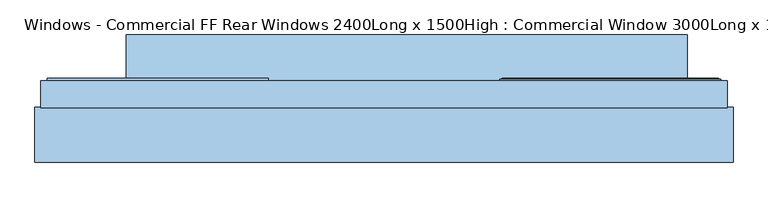
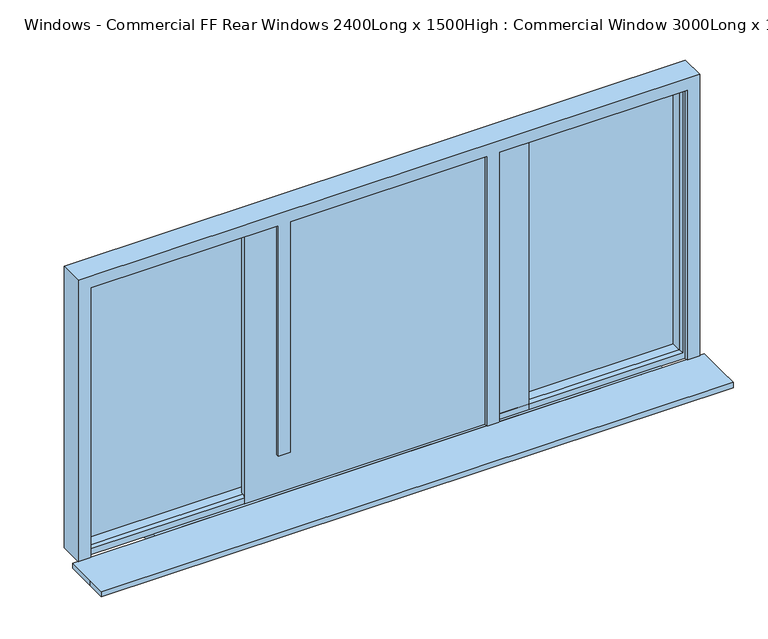
"""IFC4 building model written with IfcOpenShell, lengths in millimetres: window geometry, Windows - Commercial FF Rear Windows 2400Long x 1500High : Commercial Window 3000Long x 1500High 2."""

import ifcopenshell
import ifcopenshell.guid

model = None  # the IFC model being written
_history = None  # IfcOwnerHistory: only IFC2X3 demands one
_inside = {}  # id of a spatial element -> (the spatial element, [elements in it])
_under = {}  # id of a project, library or spatial element -> (it, [spatial elements below it])
_declared = {}  # id of a project -> (the project, [libraries it declares])
_typed = {}  # id of a type object -> (the type object, [elements of that type])
_made_of = {}  # id of a material, layer set ... -> (it, [elements and type objects made of it])


def new_model(schema):
    """Start an empty IFC model of exactly this schema.

    Asked for "IFC4X3", IfcOpenShell would pick the latest addendum, in which some entities
    have other attributes; the version numbers below select the first issue.
    IFC2X3 requires an IfcOwnerHistory on every rooted entity: one is made here for all.
    """
    global model, _history
    if schema == "IFC4X3":
        model = ifcopenshell.file(schema_version=(4, 3, 0, 0))
    else:
        model = ifcopenshell.file(schema=schema)
    _inside.clear()
    _under.clear()
    _declared.clear()
    _typed.clear()
    _made_of.clear()
    _history = None
    if model.schema == "IFC2X3":
        org = make("IfcOrganization", Name="unknown")
        user = make(
            "IfcPersonAndOrganization",
            ThePerson=make("IfcPerson", FamilyName="unknown"),
            TheOrganization=org,
        )
        app = make(
            "IfcApplication",
            ApplicationDeveloper=org,
            Version="unknown",
            ApplicationFullName="unknown",
            ApplicationIdentifier="unknown",
        )
        _history = make(
            "IfcOwnerHistory",
            OwningUser=user,
            OwningApplication=app,
            ChangeAction="ADDED",
            CreationDate=0,
        )
    return model


def make(cls, **values):
    """One entity of the class cls with the attributes given. An attribute that is None is left unset."""
    return model.create_entity(
        cls, **{name: value for name, value in values.items() if value is not None}
    )


def rooted(cls, **values):
    """An entity with a GlobalId (a new one), such as an element, a storey or a relation."""
    return make(cls, GlobalId=ifcopenshell.guid.new(), OwnerHistory=_history, **values)


def si_unit(unit_type, name, prefix=None):
    """IfcSIUnit, for example si_unit("LENGTHUNIT", "METRE", prefix="MILLI")."""
    return make("IfcSIUnit", UnitType=unit_type, Prefix=prefix, Name=name)


def assignment(units):
    """IfcUnitAssignment: the units of a project."""
    return None if units is None else make("IfcUnitAssignment", Units=units)


def point(xyz):
    """IfcCartesianPoint."""
    return None if xyz is None else make("IfcCartesianPoint", Coordinates=xyz)


def direction(xyz):
    """IfcDirection."""
    return None if xyz is None else make("IfcDirection", DirectionRatios=xyz)


def frame(location, z_axis=None, x_axis=None):
    """IfcAxis2Placement3D, a coordinate frame: its origin and axes. An axis left out is left unset."""
    return make(
        "IfcAxis2Placement3D",
        Location=point(location),
        Axis=direction(z_axis),
        RefDirection=direction(x_axis),
    )


def origin():
    """The frame at (0, 0, 0) with its axes left unset."""
    return frame((0.0, 0.0, 0.0))


def place(relative_to, where):
    """IfcLocalPlacement: puts the frame where relative to a parent placement (None: the world)."""
    return make(
        "IfcLocalPlacement", PlacementRelTo=relative_to, RelativePlacement=where
    )


def context(
    kind, dimensions, precision=None, world=None, true_north=None, identifier=None
):
    """IfcGeometricRepresentationContext, for example the 3D "Model" context."""
    return make(
        "IfcGeometricRepresentationContext",
        ContextIdentifier=identifier,
        ContextType=kind,
        CoordinateSpaceDimension=dimensions,
        Precision=precision,
        WorldCoordinateSystem=world,
        TrueNorth=true_north,
    )


def project(units=None, contexts=None):
    """IfcProject with its units and contexts."""
    return rooted(
        "IfcProject",
        Name="project",
        RepresentationContexts=contexts,
        UnitsInContext=assignment(units),
    )


def spatial(cls, under=None, at=None, **own):
    """A site, building, storey or space (cls), placed at a placement, below another one or the project."""
    s = rooted(cls, ObjectPlacement=at, **own)
    if under is not None:
        _under.setdefault(under.id(), (under, []))[1].append(s)
    return s


def polyline(points):
    """IfcPolyline through the points."""
    return make("IfcPolyline", Points=[point(p) for p in points])


def outline(outer, holes=None, kind="AREA"):
    """IfcArbitraryClosedProfileDef: a profile drawn as a closed curve; with holes, ...WithVoids."""
    if holes is None:
        return make("IfcArbitraryClosedProfileDef", ProfileType=kind, OuterCurve=outer)
    return make(
        "IfcArbitraryProfileDefWithVoids",
        ProfileType=kind,
        OuterCurve=outer,
        InnerCurves=holes,
    )


def extrude(swept, where, along, depth):
    """IfcExtrudedAreaSolid: the profile swept, set in the frame where, extruded along a direction by depth."""
    return make(
        "IfcExtrudedAreaSolid",
        SweptArea=swept,
        Position=where,
        ExtrudedDirection=direction(along),
        Depth=depth,
    )


def faces_of(points, faces, orient=None, outer=None):
    """IfcFace entities. A face is a list of loops; a loop is a list of indices into points, from 0.

    orient and outer hold one flag for each loop. By default every Orientation is true, the
    first loop of a face is its IfcFaceOuterBound and the others are IfcFaceBound.
    """
    made = []
    for i, loops in enumerate(faces):
        bounds = []
        for j, loop in enumerate(loops):
            is_outer = j == 0 if outer is None else outer[i][j]
            bounds.append(
                make(
                    "IfcFaceOuterBound" if is_outer else "IfcFaceBound",
                    Bound=make("IfcPolyLoop", Polygon=[points[k] for k in loop]),
                    Orientation=True if orient is None else orient[i][j],
                )
            )
        made.append(make("IfcFace", Bounds=bounds))
    return made


def faceted_brep(points, faces, orient=None, outer=None, voids=None):
    """IfcFacetedBrep: a solid bounded by flat faces; with voids (closed shells), ...WithVoids."""
    shared = [point(p) for p in points]
    hull = make("IfcClosedShell", CfsFaces=faces_of(shared, faces, orient, outer))
    if voids is None:
        return make("IfcFacetedBrep", Outer=hull)
    return make(
        "IfcFacetedBrepWithVoids",
        Outer=hull,
        Voids=[
            make(cls, CfsFaces=faces_of(shared, fs, o, b)) for cls, fs, o, b in voids
        ],
    )


def shape(context_of_items, identifier, shape_type, items):
    """IfcShapeRepresentation: the items that make up one representation, for example the "Body"."""
    return make(
        "IfcShapeRepresentation",
        ContextOfItems=context_of_items,
        RepresentationIdentifier=identifier,
        RepresentationType=shape_type,
        Items=items,
    )


def source(mapping_origin, context_of_items, identifier, shape_type, items):
    """IfcRepresentationMap: a shape defined once, which mapped items show again and again."""
    return make(
        "IfcRepresentationMap",
        MappingOrigin=mapping_origin,
        MappedRepresentation=shape(context_of_items, identifier, shape_type, items),
    )


def transform(
    local_origin,
    x_axis=None,
    y_axis=None,
    z_axis=None,
    scale=None,
    scale2=None,
    scale3=None,
    uniform=True,
):
    """IfcCartesianTransformationOperator3D, or its non-uniform kind. x_axis, y_axis, z_axis: its Axis1, 2, 3."""
    if uniform:
        return make(
            "IfcCartesianTransformationOperator3D",
            Axis1=direction(x_axis),
            Axis2=direction(y_axis),
            LocalOrigin=point(local_origin),
            Scale=scale,
            Axis3=direction(z_axis),
        )
    return make(
        "IfcCartesianTransformationOperator3DnonUniform",
        Axis1=direction(x_axis),
        Axis2=direction(y_axis),
        LocalOrigin=point(local_origin),
        Scale=scale,
        Axis3=direction(z_axis),
        Scale2=scale2,
        Scale3=scale3,
    )


def mapped(mapping_source, mapping_target):
    """IfcMappedItem: shows the shape of a source again, moved by a transform."""
    return make(
        "IfcMappedItem", MappingSource=mapping_source, MappingTarget=mapping_target
    )


def made_of(thing, what):
    """Note that an element or type object is made of a material, layer set ...; save() writes the relation."""
    if what is not None:
        _made_of.setdefault(what.id(), (what, []))[1].append(thing)
    return thing


def element(
    cls,
    number,
    at=None,
    inside=None,
    cuts=None,
    type_object=None,
    material=None,
    context=None,
    identifier="Body",
    shape_type=None,
    held_by="IfcProductDefinitionShape",
    body=None,
    shapes=None,
    **own,
):
    """One element of the class cls, such as IfcWall. Its Tag is "e" and its number.

    at: its placement. inside: the storey or other place that contains it. cuts: it is an
    opening in that element (IfcRelVoidsElement). A single representation is given by context,
    identifier, shape_type and body (its items); several are given by shapes. held_by: the class
    of the entity that holds the representations. save() writes the other relations.
    """
    e = rooted(cls, Tag="e%d" % number, ObjectPlacement=at, **own)
    if body is not None:
        shapes = [shape(context, identifier, shape_type, body)]
    if shapes is not None:
        e.Representation = make(held_by, Representations=shapes)
    if inside is not None:
        _inside.setdefault(inside.id(), (inside, []))[1].append(e)
    if cuts is not None:
        rooted(
            "IfcRelVoidsElement", RelatingBuildingElement=cuts, RelatedOpeningElement=e
        )
    if type_object is not None:
        _typed.setdefault(type_object.id(), (type_object, []))[1].append(e)
    return made_of(e, material)


def aggregate(whole, parts):
    """IfcRelAggregates: a whole, such as a stair, and the parts it consists of."""
    return rooted("IfcRelAggregates", RelatingObject=whole, RelatedObjects=parts)


def save(model, path):
    """Write the relations noted so far, then the file.

    IfcRelAggregates (storeys below a building ...), IfcRelContainedInSpatialStructure (elements
    in a storey), IfcRelDefinesByType, IfcRelAssociatesMaterial and IfcRelDeclares: one each for
    every whole, place, type object, material and project.
    """
    for whole, parts in _under.values():
        aggregate(whole, parts)
    for where, things in _inside.values():
        rooted(
            "IfcRelContainedInSpatialStructure",
            RelatedElements=things,
            RelatingStructure=where,
        )
    for kind, things in _typed.values():
        rooted("IfcRelDefinesByType", RelatedObjects=things, RelatingType=kind)
    for what, things in _made_of.values():
        rooted("IfcRelAssociatesMaterial", RelatedObjects=things, RelatingMaterial=what)
    for by, libraries in _declared.values():
        rooted("IfcRelDeclares", RelatingContext=by, RelatedDefinitions=libraries)
    model.write(path)


def windows_commercial_ff_rear_windows_2400long_x_1500high_ec56d910(model_context):
    return source(origin(), model_context, "Body", "SolidModel", [
        extrude(outline(polyline([(-2260.0, -231.5434322), (-2260.0, -138.5434322), (-2260.0, 8.4565678), (790.0, 8.4565678), (790.0, -138.5434322), (790.0, -231.5434322), (-2260.0, -231.5434322)])), frame((0.0, 0.0, 636.5715519), z_axis=(0.0, 0.0, 1.0), x_axis=(1.0, 0.0, 0.0)), (0.0, 0.0, 1.0), 26.4284481),
        extrude(outline(polyline([(695.0, 87.4565678), (-190.0, 87.4565678), (-190.0, 111.4565678), (695.0, 111.4565678), (695.0, 87.4565678)])), frame((0.0, 0.0, 693.0), z_axis=(0.0, 0.0, 1.0), x_axis=(1.0, 0.0, 0.0)), (0.0, 0.0, 1.0), 1337.0),
        extrude(outline(polyline([(-1420.0, 47.4565678), (-50.0, 47.4565678), (-50.0, 23.4565678), (-1420.0, 23.4565678), (-1420.0, 47.4565678)])), frame((0.0, 0.0, 663.0), z_axis=(0.0, 0.0, 1.0), x_axis=(1.0, 0.0, 0.0)), (0.0, 0.0, 1.0), 1397.0),
        extrude(outline(polyline([(-1280.0, 87.4565678), (-2165.0, 87.4565678), (-2165.0, 111.4565678), (-1280.0, 111.4565678), (-1280.0, 87.4565678)])), frame((0.0, 0.0, 693.0), z_axis=(0.0, 0.0, 1.0), x_axis=(1.0, 0.0, 0.0)), (0.0, 0.0, 1.0), 1337.0),
        faceted_brep([(-2235.0, 5.4565678, 663.0), (-2175.0, 5.4565678, 663.0), (-2175.0, 5.4565678, 2040.0), (-1268.0, 5.4565678, 2040.0), (-1268.0, 5.4565678, 863.0), (-1210.0, 5.4565678, 863.0), (-1210.0, 5.4565678, 2040.0), (-260.0, 5.4565678, 2040.0), (-260.0, 5.4565678, 663.0), (-202.0, 5.4565678, 663.0), (-202.0, 5.4565678, 2040.0), (705.0, 5.4565678, 2040.0), (705.0, 5.4565678, 663.0), (765.0, 5.4565678, 663.0), (765.0, 5.4565678, 2100.0), (-2235.0, 5.4565678, 2100.0), (-2235.0, 123.4565678, 663.0), (-2235.0, 123.4565678, 2100.0), (-2195.0, 123.4565678, 663.0), (765.0, 123.4565678, 2100.0), (765.0, 123.4565678, 663.0), (725.0, 123.4565678, 663.0), (725.0, 123.4565678, 2060.0), (-220.0, 123.4565678, 2060.0), (-220.0, 123.4565678, 663.0), (-260.0, 123.4565678, 663.0), (-260.0, 123.4565678, 2060.0), (-1210.0, 123.4565678, 2060.0), (-1210.0, 123.4565678, 863.0), (-1250.0, 123.4565678, 863.0), (-1250.0, 123.4565678, 2060.0), (-2195.0, 123.4565678, 2060.0), (-2195.0, 23.4565678, 663.0), (-2195.0, 23.4565678, 2060.0), (-2175.0, 23.4565678, 663.0), (-1250.0, 23.4565678, 2060.0), (-1250.0, 23.4565678, 863.0), (-1268.0, 23.4565678, 863.0), (-1268.0, 23.4565678, 2040.0), (-2175.0, 23.4565678, 2040.0), (725.0, 23.4565678, 2060.0), (725.0, 23.4565678, 663.0), (705.0, 23.4565678, 663.0), (705.0, 23.4565678, 2040.0), (-202.0, 23.4565678, 2040.0), (-202.0, 23.4565678, 663.0), (-220.0, 23.4565678, 663.0), (-220.0, 23.4565678, 2060.0), (-1210.0, 23.4565678, 863.0), (-1220.0, 23.4565678, 863.0), (-1220.0, 23.4565678, 2060.0), (-250.0, 23.4565678, 2060.0), (-250.0, 23.4565678, 663.0), (-260.0, 23.4565678, 663.0), (-260.0, 23.4565678, 2040.0), (-1210.0, 23.4565678, 2040.0), (-1210.0, 47.4565678, 2060.0), (-260.0, 47.4565678, 2060.0), (-250.0, 47.4565678, 2060.0), (-1220.0, 47.4565678, 2060.0), (-1210.0, 47.4565678, 863.0), (-1220.0, 47.4565678, 863.0), (-250.0, 47.4565678, 663.0), (-260.0, 47.4565678, 663.0), (-260.0, 73.4565678, 663.0), (-220.0, 73.4565678, 663.0), (-202.0, 8.4565678, 663.0), (-260.0, 8.4565678, 663.0), (590.0, 323.4565678, 600.0), (590.0, 8.4565678, 600.0), (-1860.0, 8.4565678, 600.0), (-1860.0, 323.4565678, 600.0), (590.0, 323.4565678, 637.0666405), (-1860.0, 323.4565678, 637.0666405), (590.0, 73.4565678, 649.0962075), (-1860.0, 73.4565678, 649.0962075), (590.0, 8.4565678, 663.0), (590.0, 73.4565678, 663.0), (-1860.0, 73.4565678, 663.0), (-1860.0, 8.4565678, 663.0)], [[[0, 1, 2, 3, 4, 5, 6, 7, 8, 9, 10, 11, 12, 13, 14, 15]], [[16, 0, 15, 17]], [[18, 16, 17, 19, 20, 21, 22, 23, 24, 25, 26, 27, 28, 29, 30, 31]], [[32, 18, 31, 33]], [[34, 32, 33, 35, 36, 37, 38, 39]], [[40, 41, 42, 43, 44, 45, 46, 47]], [[48, 49, 50, 51, 52, 53, 54, 55]], [[1, 34, 39, 2]], [[15, 14, 19, 17]], [[33, 31, 30, 35]], [[22, 40, 47, 23]], [[56, 27, 26, 57, 58, 51, 50, 59]], [[2, 39, 38, 3]], [[43, 11, 10, 44]], [[6, 55, 54, 7]], [[14, 13, 20, 19]], [[22, 21, 41, 40]], [[12, 11, 43, 42]], [[5, 48, 55, 6]], [[37, 4, 3, 38]], [[29, 36, 35, 30]], [[60, 28, 27, 56]], [[61, 60, 56, 59]], [[49, 61, 59, 50]], [[58, 62, 52, 51]], [[62, 58, 57, 63]], [[63, 57, 26, 25, 64]], [[24, 23, 47, 46, 65]], [[10, 9, 66, 45, 44]], [[8, 7, 54, 53, 67]], [[68, 69, 70, 71]], [[72, 68, 71, 73]], [[74, 72, 73, 75]], [[76, 77, 65, 46, 45, 66]], [[78, 79, 67, 53, 52, 62, 63, 64]], [[1, 0, 16, 18, 32, 34]], [[13, 12, 42, 41, 21, 20]], [[48, 5, 4, 37, 36, 29, 28, 60, 61, 49]], [[25, 24, 65, 64]], [[9, 8, 67, 66]], [[76, 69, 68, 72, 74, 77]], [[79, 78, 75, 73, 71, 70]], [[77, 74, 75, 78, 64, 65]], [[69, 76, 66, 67, 79, 70]]]),
        faceted_brep([(-1250.0, 23.4565678, 2060.0), (-1250.0, 93.4565678, 2060.0), (-2195.0, 93.4565678, 2060.0), (-2195.0, 23.4565678, 2060.0), (-1290.0, 37.9494677, 2020.0), (-1279.8519623, 23.4565678, 2030.1480377), (-2165.1480377, 23.4565678, 2030.1480377), (-2155.0, 37.9494677, 2020.0), (-1290.0, 87.4565678, 2020.0), (-2155.0, 87.4565678, 2020.0), (-1280.0, 111.4565678, 2030.0), (-1280.0, 87.4565678, 2030.0), (-2165.0, 87.4565678, 2030.0), (-2165.0, 111.4565678, 2030.0), (-1290.0, 129.2300705, 2020.0), (-1290.0, 111.4565678, 2020.0), (-2155.0, 111.4565678, 2020.0), (-2155.0, 129.2300705, 2020.0), (-1271.1854344, 135.0035732, 2038.8145656), (-2173.8145656, 135.0035732, 2038.8145656), (-2195.0, 93.4565678, 663.0), (-2195.0, 23.4565678, 663.0), (-2165.1480377, 23.4565678, 692.8519623), (-2155.0, 37.9494677, 703.0), (-2155.0, 87.4565678, 703.0), (-2165.0, 87.4565678, 693.0), (-2165.0, 111.4565678, 693.0), (-2155.0, 111.4565678, 703.0), (-2155.0, 129.2300705, 703.0), (-2173.8145656, 135.0035732, 684.1854344), (-1250.0, 93.4565678, 663.0), (-1250.0, 23.4565678, 663.0), (-1279.8519623, 23.4565678, 692.8519623), (-1290.0, 37.9494677, 703.0), (-1290.0, 87.4565678, 703.0), (-1280.0, 87.4565678, 693.0), (-1280.0, 111.4565678, 693.0), (-1290.0, 111.4565678, 703.0), (-1290.0, 129.2300705, 703.0), (-1271.1854344, 135.0035732, 684.1854344), (-1240.0, 135.0035732, 653.0), (-2205.0, 135.0035732, 653.0), (-2205.0, 135.0035732, 2070.0), (-1240.0, 135.0035732, 2070.0), (-1240.0, 93.4565678, 2070.0), (-2205.0, 93.4565678, 2070.0), (-2205.0, 93.4565678, 653.0), (-1240.0, 93.4565678, 653.0)], [[[0, 1, 2, 3]], [[4, 5, 6, 7]], [[8, 4, 7, 9]], [[10, 11, 12, 13]], [[14, 15, 16, 17]], [[18, 14, 17, 19]], [[3, 2, 20, 21]], [[7, 6, 22, 23]], [[9, 7, 23, 24]], [[13, 12, 25, 26]], [[17, 16, 27, 28]], [[19, 17, 28, 29]], [[21, 20, 30, 31]], [[0, 3, 21, 31], [32, 22, 6, 5]], [[23, 22, 32, 33]], [[24, 23, 33, 34]], [[35, 25, 12, 11], [8, 9, 24, 34]], [[26, 25, 35, 36]], [[10, 13, 26, 36], [37, 27, 16, 15]], [[28, 27, 37, 38]], [[29, 28, 38, 39]], [[40, 41, 42, 43], [18, 19, 29, 39]], [[30, 1, 0, 31]], [[33, 32, 5, 4]], [[34, 33, 4, 8]], [[36, 35, 11, 10]], [[38, 37, 15, 14]], [[39, 38, 14, 18]], [[44, 43, 42, 45]], [[45, 42, 41, 46]], [[46, 41, 40, 47]], [[47, 40, 43, 44]], [[45, 46, 47, 44], [1, 30, 20, 2]]]),
        faceted_brep([(-230.0, 87.4565678, 2070.0), (-230.0, 129.2300705, 2070.0), (-230.0, 129.2300705, 653.0), (-230.0, 87.4565678, 653.0), (-220.0, 23.4565678, 2060.0), (-220.0, 87.4565678, 2060.0), (-220.0, 87.4565678, 663.0), (-220.0, 23.4565678, 663.0), (-180.0, 37.9494677, 2020.0), (-190.1480377, 23.4565678, 2030.1480377), (-190.1480377, 23.4565678, 692.8519623), (-180.0, 37.9494677, 703.0), (-180.0, 87.4565678, 2020.0), (-180.0, 87.4565678, 703.0), (-190.0, 111.4565678, 2030.0), (-190.0, 87.4565678, 2030.0), (-190.0, 87.4565678, 693.0), (-190.0, 111.4565678, 693.0), (-180.0, 129.2300705, 2020.0), (-180.0, 111.4565678, 2020.0), (-180.0, 111.4565678, 703.0), (-180.0, 129.2300705, 703.0), (-197.4457548, 135.0035732, 2037.4457548), (-197.4457548, 135.0035732, 685.5542452), (-219.2153903, 135.0035732, 2059.2153903), (-219.2153903, 135.0035732, 663.7846097), (735.0, 129.2300705, 653.0), (735.0, 87.4565678, 653.0), (725.0, 87.4565678, 663.0), (725.0, 23.4565678, 663.0), (695.1480377, 23.4565678, 692.8519623), (685.0, 37.9494677, 703.0), (685.0, 87.4565678, 703.0), (695.0, 87.4565678, 693.0), (695.0, 111.4565678, 693.0), (685.0, 111.4565678, 703.0), (685.0, 129.2300705, 703.0), (702.4457548, 135.0035732, 685.5542452), (724.2153903, 135.0035732, 663.7846097), (735.0, 129.2300705, 2070.0), (735.0, 87.4565678, 2070.0), (725.0, 87.4565678, 2060.0), (725.0, 23.4565678, 2060.0), (695.1480377, 23.4565678, 2030.1480377), (685.0, 37.9494677, 2020.0), (685.0, 87.4565678, 2020.0), (695.0, 87.4565678, 2030.0), (695.0, 111.4565678, 2030.0), (685.0, 111.4565678, 2020.0), (685.0, 129.2300705, 2020.0), (702.4457548, 135.0035732, 2037.4457548), (724.2153903, 135.0035732, 2059.2153903)], [[[0, 1, 2, 3]], [[4, 5, 6, 7]], [[8, 9, 10, 11]], [[12, 8, 11, 13]], [[14, 15, 16, 17]], [[18, 19, 20, 21]], [[22, 18, 21, 23]], [[1, 24, 25, 2]], [[3, 2, 26, 27]], [[7, 6, 28, 29]], [[11, 10, 30, 31]], [[13, 11, 31, 32]], [[17, 16, 33, 34]], [[21, 20, 35, 36]], [[23, 21, 36, 37]], [[2, 25, 38, 26]], [[27, 26, 39, 40]], [[29, 28, 41, 42]], [[31, 30, 43, 44]], [[32, 31, 44, 45]], [[34, 33, 46, 47]], [[36, 35, 48, 49]], [[37, 36, 49, 50]], [[26, 38, 51, 39]], [[40, 39, 1, 0]], [[42, 41, 5, 4]], [[7, 29, 42, 4], [9, 43, 30, 10]], [[44, 43, 9, 8]], [[45, 44, 8, 12]], [[15, 46, 33, 16], [13, 32, 45, 12]], [[47, 46, 15, 14]], [[17, 34, 47, 14], [19, 48, 35, 20]], [[49, 48, 19, 18]], [[50, 49, 18, 22]], [[24, 51, 38, 25], [23, 37, 50, 22]], [[39, 51, 24, 1]], [[3, 27, 40, 0], [5, 41, 28, 6]]]),
    ])


if __name__ == "__main__":
    model = new_model("IFC4")
    model_context = context("Model", 3, world=origin())
    ifc_project = project(units=[si_unit("LENGTHUNIT", "METRE", prefix="MILLI")], contexts=[model_context])
    site = spatial("IfcSite", under=ifc_project)
    building = spatial("IfcBuilding", under=site)
    placement = place(None, origin())
    windows_commercial_ff_rear_windows_2400long_x_1500high_shape = windows_commercial_ff_rear_windows_2400long_x_1500high_ec56d910(model_context)
    element("IfcWindow", 1, ObjectType="Windows - Commercial FF Rear Windows 2400Long x 1500High : Commercial Window 3000Long x 1500High 2", at=placement, inside=building, context=model_context, shape_type="MappedRepresentation", body=[
        mapped(windows_commercial_ff_rear_windows_2400long_x_1500high_shape, transform((0.0, 0.0, 0.0), x_axis=(1.0, 0.0, 0.0), y_axis=(0.0, 1.0, 0.0), z_axis=(0.0, 0.0, 1.0))),
    ])
    save(model, "model.ifc")

# Revit data of these elements
# Type "Windows - Commercial FF Rear Windows 2400Long x 1500High : Commercial Window 3000Long x 1500High 2"
#   Type Mark = "67"
#   Operation = "Triple Panel Vertical"
#   Description = "Double Glazed First Floor Window"
#   Manufacturer = "aluminium Co"
#   Keynote = "L10"
#   Wrap Layers (Ext) from Ext = 100 mm
#   Wrap Layers (Int) from Ext = 177.5 mm
#   Window Board Projection = 25 mm
#   Window Board Extension = 25 mm
#   Visual Light Transmittance = 0.9
#   Solar Heat Gain Coefficient = 0.78
#   Rough Width = 3000 mm
#   Rough Height = 1500 mm
#   Height = 1500 mm
#   Width = 3000 mm
#   Heat Transfer Coefficient (U) = 3.6886 W/(m²·K)
#   Glazing Thickness = 24 mm
#   FrameOffset - External = 100 mm
#   Frame Depth = 100 mm
#   Default Head Height = 2100 mm
#   Cill Depth = 200 mm
#   Cavity Closer Width = 100 mm
#   Cavity Closer Offset from Ext = 130 mm
#   Cavity Closer Depth = 85 mm
#   Vis - Cavity Closers = yes
#   Define Thermal Properties by = 1
#   Material Trim = Window Frame
#   Material Glass = Glass
#   Material Frame = Window Frame
#   Construction Type Id = ""
#   Wall Closure = (empty or 0)
#   Analytic Construction = (empty or 0)
# Element 1 (IfcWindow, "Windows - Commercial FF Rear Windows 2400Long x 1500High : Commercial Window 3000Long x 1500High 2")
#   Materials on its faces: "Window Frame", "Glass"
# Materials
#   "Window Frame": class "Miscellaneous", colour RGB 249 249 249, transparency 0, Keynote = "L10"
#   "Glass": class "Glass", colour RGB 0 128 192, transparency 0.9, Description = "Soda Lime Glass", Cost = 0
